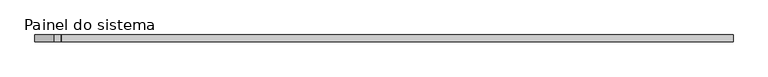
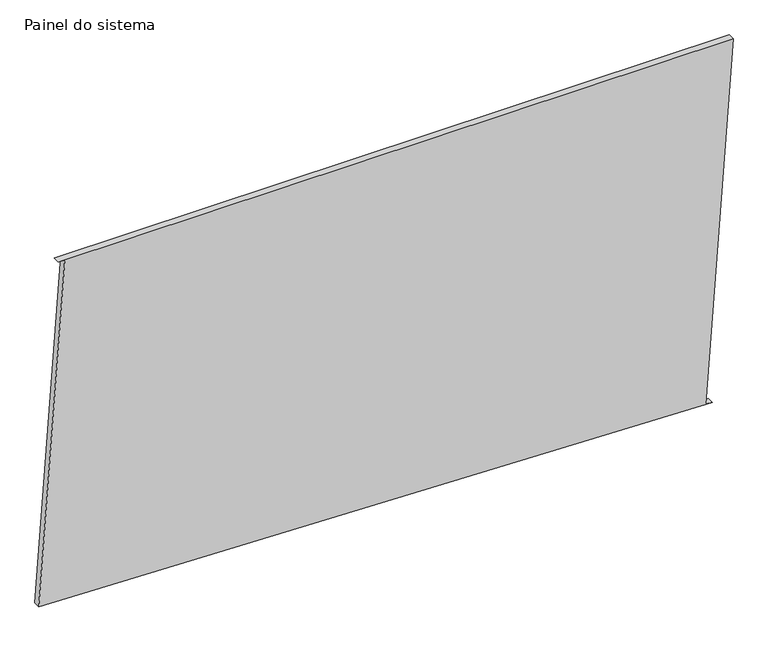
"""IFC4 building model written with IfcOpenShell, lengths in millimetres: plate geometry, Painel do sistema : Envidraçado."""

from ifc_helpers import new_model, si_unit, frame, origin, place, context, project, spatial, polyline, outline, extrude, source, transform, mapped, element, save


def painel_do_sistema_b97b7537(model_context):
    return source(origin(), model_context, "Body", "SweptSolid", [
        extrude(outline(polyline([(0.0, 1235.0405513), (1.8159485, 1210.1065919), (1428.1770246, 1313.9889395), (1428.1770246, -1240.3877018), (1426.3610761, -1215.4537424), (73.4192812, -1313.9889395), (0.0, 1235.0405513)])), frame((0.0, 24.5, 0.0), z_axis=(0.0, 1.0, 0.0), x_axis=(0.0, 0.0, 1.0)), (0.0, 0.0, 1.0), 25.0),
    ])


if __name__ == "__main__":
    model = new_model("IFC4")
    model_context = context("Model", 3, world=origin())
    ifc_project = project(units=[si_unit("LENGTHUNIT", "METRE", prefix="MILLI")], contexts=[model_context])
    site = spatial("IfcSite", under=ifc_project)
    building = spatial("IfcBuilding", under=site)
    placement = place(None, origin())
    painel_do_sistema_shape = painel_do_sistema_b97b7537(model_context)
    element("IfcPlate", 1, ObjectType="Painel do sistema : Envidraçado", at=placement, inside=building, context=model_context, shape_type="MappedRepresentation", body=[
        mapped(painel_do_sistema_shape, transform((0.0, 0.0, 0.0), x_axis=(1.0, 0.0, 0.0), y_axis=(0.0, 1.0, 0.0), z_axis=(0.0, 0.0, 1.0))),
    ])
    save(model, "model.ifc")

# Revit data of these elements
# Type "Painel do sistema : Envidraçado"
#   Construction Type Id = "GSP4R"
#   Analytic Construction = "Vidraça única Pilkington 1/8 pol"
#   Visual Light Transmittance = 0.9
#   Solar Heat Gain Coefficient = 0.86
#   Heat Transfer Coefficient (U) = 6.7069 W/(m²·K)
# Element 1 (IfcPlate, "Painel do sistema : Envidraçado")
#   Materials on its faces: "Vidro"
# Materials
#   "Vidro": class "Vidro", colour RGB 0 128 192, transparency 0.9, Description = "Vidro de sílica", Cost = 0
